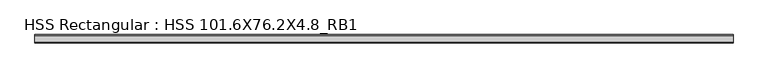
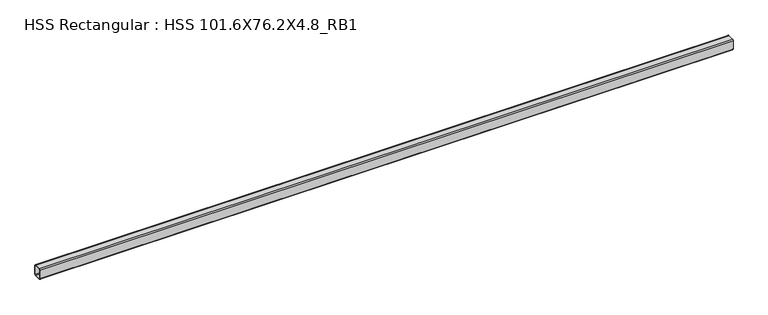
"""IFC4 building model written with IfcOpenShell, lengths in millimetres: beam geometry, HSS Rectangular : HSS 101.6X76.2X4.8_RB1."""

from ifc_helpers import new_model, si_unit, point, frame, frame_2d, origin, place, context, project, spatial, polyline, circle_curve, trimmed, segment, composite_curve, outline, extrude, source, transform, mapped, element, save


def hss_rectangular_hss_101_6x76_2x4_8_rb1_ef47b5ec(model_context):
    return source(origin(), model_context, "Body", "SweptSolid", [
        extrude(outline(composite_curve([segment(polyline([(38.1, 41.275), (38.1, -41.275)]), True, "CONTINUOUS"), segment(trimmed(circle_curve(frame_2d((28.575, -41.275)), 9.525), [point((38.1, -41.275))], [point((28.575, -50.8))], False, "CARTESIAN"), True, "CONTINUOUS"), segment(polyline([(28.575, -50.8), (-28.575, -50.8)]), True, "CONTINUOUS"), segment(trimmed(circle_curve(frame_2d((-28.575, -41.275)), 9.525), [point((-28.575, -50.8))], [point((-38.1, -41.275))], False, "CARTESIAN"), True, "CONTINUOUS"), segment(polyline([(-38.1, -41.275), (-38.1, 41.275)]), True, "CONTINUOUS"), segment(trimmed(circle_curve(frame_2d((-28.575, 41.275)), 9.525), [point((-38.1, 41.275))], [point((-28.575, 50.8))], False, "CARTESIAN"), True, "CONTINUOUS"), segment(polyline([(-28.575, 50.8), (28.575, 50.8)]), True, "CONTINUOUS"), segment(trimmed(circle_curve(frame_2d((28.575, 41.275)), 9.525), [point((28.575, 50.8))], [point((38.1, 41.275))], False, "CARTESIAN"), True, "CONTINUOUS")], self_intersect=False), holes=[composite_curve([segment(trimmed(circle_curve(frame_2d((-28.575, 41.275)), 4.7625), [point((-28.575, 46.0375))], [point((-33.3375, 41.275))], True, "CARTESIAN"), True, "CONTINUOUS"), segment(polyline([(-33.3375, 41.275), (-33.3375, -41.275)]), True, "CONTINUOUS"), segment(trimmed(circle_curve(frame_2d((-28.575, -41.275)), 4.7625), [point((-33.3375, -41.275))], [point((-28.575, -46.0375))], True, "CARTESIAN"), True, "CONTINUOUS"), segment(polyline([(-28.575, -46.0375), (28.575, -46.0375)]), True, "CONTINUOUS"), segment(trimmed(circle_curve(frame_2d((28.575, -41.275)), 4.7625), [point((28.575, -46.0375))], [point((33.3375, -41.275))], True, "CARTESIAN"), True, "CONTINUOUS"), segment(polyline([(33.3375, -41.275), (33.3375, 41.275)]), True, "CONTINUOUS"), segment(trimmed(circle_curve(frame_2d((28.575, 41.275)), 4.7625), [point((33.3375, 41.275))], [point((28.575, 46.0375))], True, "CARTESIAN"), True, "CONTINUOUS"), segment(polyline([(28.575, 46.0375), (-28.575, 46.0375)]), True, "CONTINUOUS")], self_intersect=False)]), frame((-7639.3766079, 0.0, 0.0), z_axis=(1.0, 0.0, 0.0), x_axis=(0.0, 1.0, 0.0)), (0.0, 0.0, 1.0), 6368.0912391),
    ])


if __name__ == "__main__":
    model = new_model("IFC4")
    model_context = context("Model", 3, world=origin())
    ifc_project = project(units=[si_unit("LENGTHUNIT", "METRE", prefix="MILLI")], contexts=[model_context])
    site = spatial("IfcSite", under=ifc_project)
    building = spatial("IfcBuilding", under=site)
    placement = place(None, origin())
    hss_rectangular_hss_101_6x76_2x4_8_rb1_shape = hss_rectangular_hss_101_6x76_2x4_8_rb1_ef47b5ec(model_context)
    element("IfcBeam", 1, ObjectType="HSS Rectangular : HSS 101.6X76.2X4.8_RB1", at=placement, inside=building, context=model_context, shape_type="MappedRepresentation", body=[
        mapped(hss_rectangular_hss_101_6x76_2x4_8_rb1_shape, transform((0.0, 0.0, 0.0), x_axis=(1.0, 0.0, 0.0), y_axis=(0.0, 1.0, 0.0), z_axis=(0.0, 0.0, 1.0))),
    ])
    save(model, "model.ifc")

# Revit data of these elements
# Type "HSS Rectangular : HSS 101.6X76.2X4.8_RB1"
#   Section Name Key = "HSS 4X3X3/16"
#   Assembly Code = "B10"
#   Width = 7.62 cm
#   Wall Nominal Thickness = 0.4763 cm
#   Wall Design Thickness = 0.442 cm
#   Torsional Moment of Inertia = 260.561 cm⁴
#   Torsional Modulus = 61.2876 cm³
#   Section Area = 14.4516 cm²
#   Plastic Modulus weak axis = 40.3122 cm³
#   Plastic Modulus strong axis = 49.1612 cm³
#   Perimeter = 0.881482 m²/m
#   Outer Fillet = 0.9525 cm
#   Nominal Weight = 12.1285 kgf/m
#   Moment of Inertia weak axis = 131.529 cm⁴
#   Moment of Inertia strong axis = 205.202 cm⁴
#   Inner Fillet = 0.4763 cm
#   Height = 10.16 cm
#   Elastic Modulus weak axis = 34.4128 cm³
#   Elastic Modulus strong axis = 40.476 cm³
#   Centroid Vertical = 5.08 cm
#   Centroid Horizontal = 3.81 cm
#   Length [instance default] = 1524 mm
#   Structural Material [instance default] = Steel ASTM A500, Grade B, Rectangular and Square
#   Principal Axes Angle = 0
# Element 1 (IfcBeam, "HSS Rectangular : HSS 101.6X76.2X4.8_RB1")
#   Structural Material = Steel ASTM A992
#   Materials on its faces: "Steel ASTM A992"
# Materials
#   "Steel ASTM A500, Grade B, Rectangular and Square": class "Metal", colour RGB 199 199 199, transparency 0, Description = "Carbon steel", Cost = 0
#   "Steel ASTM A992": class "Metal", colour RGB 199 199 199, transparency 0, Description = "Structural steel 50ksi", Cost = 0
